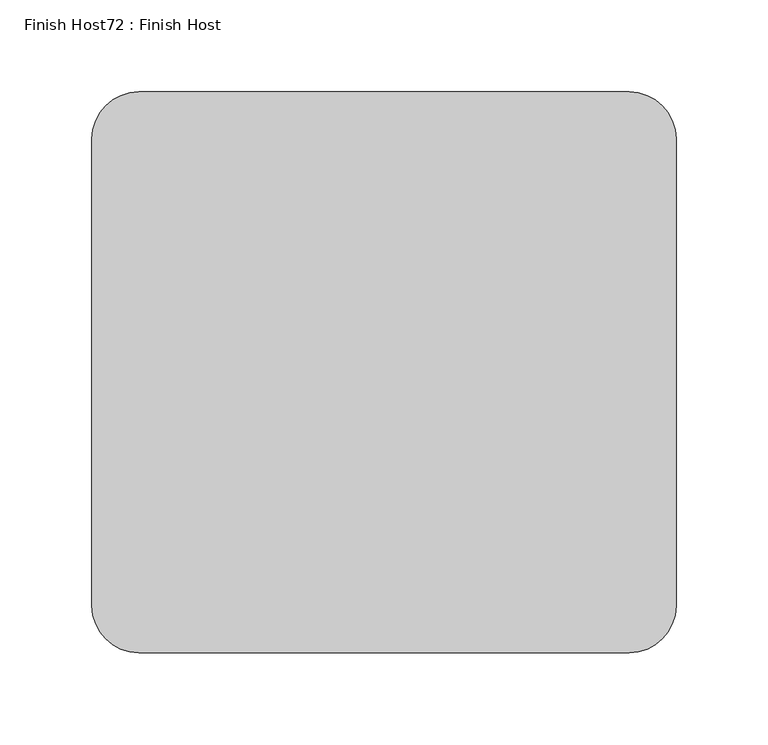
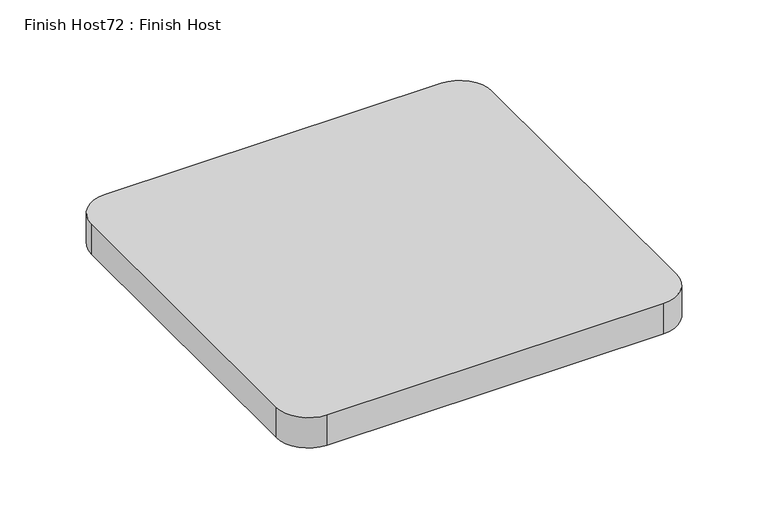
"""IFC4 building model written with IfcOpenShell, lengths in millimetres: proxy geometry, Finish Host72 : Finish Host."""

from ifc_helpers import new_model, si_unit, point, frame_2d, origin, origin_with_axes, place, context, project, spatial, polyline, circle_curve, trimmed, segment, composite_curve, outline, extrude, source, transform, mapped, element, save


def finish_host72_finish_host_cbe81b9a(model_context):
    return source(origin(), model_context, "Body", "SweptSolid", [
        extrude(outline(composite_curve([segment(polyline([(-17114.188729, 3916.6189424), (-17114.188729, 4170.6189424)]), True, "CONTINUOUS"), segment(trimmed(circle_curve(frame_2d((-17088.788729, 4170.6189424)), 25.4), [point((-17114.188729, 4170.6189424))], [point((-17088.788729, 4196.0189424))], False, "CARTESIAN"), True, "CONTINUOUS"), segment(polyline([(-17088.788729, 4196.0189424), (-16822.088729, 4196.0189424)]), True, "CONTINUOUS"), segment(trimmed(circle_curve(frame_2d((-16822.088729, 4170.6189424)), 25.4), [point((-16822.088729, 4196.0189424))], [point((-16796.688729, 4170.6189424))], False, "CARTESIAN"), True, "CONTINUOUS"), segment(polyline([(-16796.688729, 4170.6189424), (-16796.688729, 3916.6189424)]), True, "CONTINUOUS"), segment(trimmed(circle_curve(frame_2d((-16822.088729, 3916.6189424)), 25.4), [point((-16796.688729, 3916.6189424))], [point((-16822.088729, 3891.2189424))], False, "CARTESIAN"), True, "CONTINUOUS"), segment(polyline([(-16822.088729, 3891.2189424), (-17088.788729, 3891.2189424)]), True, "CONTINUOUS"), segment(trimmed(circle_curve(frame_2d((-17088.788729, 3916.6189424)), 25.4), [point((-17088.788729, 3891.2189424))], [point((-17114.188729, 3916.6189424))], False, "CARTESIAN"), True, "CONTINUOUS")], self_intersect=False)), origin_with_axes(), (0.0, 0.0, 1.0), 25.4),
    ])


if __name__ == "__main__":
    model = new_model("IFC4")
    model_context = context("Model", 3, world=origin())
    ifc_project = project(units=[si_unit("LENGTHUNIT", "METRE", prefix="MILLI")], contexts=[model_context])
    site = spatial("IfcSite", under=ifc_project)
    building = spatial("IfcBuilding", under=site)
    placement = place(None, origin())
    finish_host72_finish_host_shape = finish_host72_finish_host_cbe81b9a(model_context)
    element("IfcBuildingElementProxy", 1, Name="Finish Host72 : Finish Host", ObjectType="Finish Host72 : Finish Host", at=placement, inside=building, context=model_context, shape_type="MappedRepresentation", body=[
        mapped(finish_host72_finish_host_shape, transform((0.0, 0.0, 0.0), x_axis=(1.0, 0.0, 0.0), y_axis=(0.0, 1.0, 0.0), z_axis=(0.0, 0.0, 1.0))),
    ])
    save(model, "model.ifc")

# Revit data of these elements
# Type "Finish Host72 : Finish Host"
#   Countertop Material = Plastic - Teknion - E - Ebony
# Element 1 (IfcBuildingElementProxy, "Finish Host72 : Finish Host")
#   Materials on its faces: "Plastic - Teknion - E - Ebony"
# Materials
#   "Plastic - Teknion - E - Ebony": class "Plastic", colour RGB 5 5 5, transparency 0, Model = "E", Manufacturer = "Teknion Studio", URL = "http://www.teknion.com/", Description = "Ebony", Cost = 0
